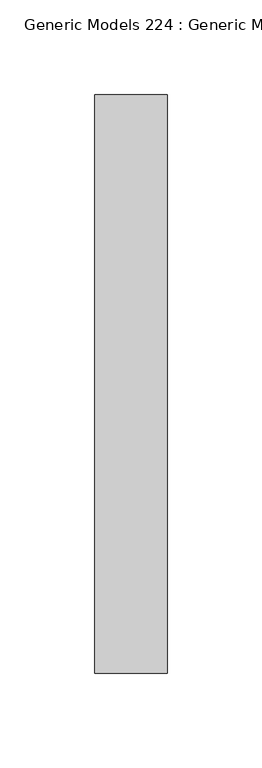
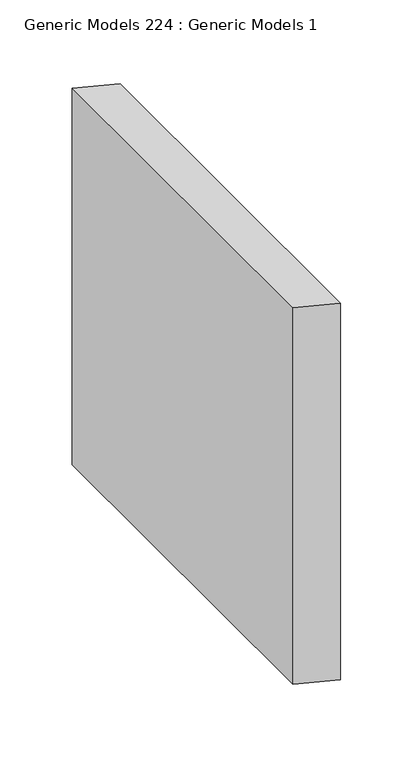
"""IFC4 building model written with IfcOpenShell, lengths in millimetres: proxy geometry, Generic Models 224 : Generic Models 1."""

from ifc_helpers import new_model, si_unit, frame, origin, place, context, project, spatial, polyline, outline, extrude, source, transform, mapped, element, save


def generic_models_224_generic_models_1_b6cca37e(model_context):
    return source(origin(), model_context, "Body", "SweptSolid", [
        extrude(outline(polyline([(126823.3589392, -31196.2089809), (126813.831285, -31158.1089809), (127131.3569728, -31158.1089809), (127140.8819728, -31196.2089809), (126823.3589392, -31196.2089809)])), frame((0.0, 21665.9639348, 0.0), z_axis=(0.0, 1.0, 0.0), x_axis=(0.0, 0.0, 1.0)), (0.0, 0.0, 1.0), 304.8),
    ])


if __name__ == "__main__":
    model = new_model("IFC4")
    model_context = context("Model", 3, world=origin())
    ifc_project = project(units=[si_unit("LENGTHUNIT", "METRE", prefix="MILLI")], contexts=[model_context])
    site = spatial("IfcSite", under=ifc_project)
    building = spatial("IfcBuilding", under=site)
    placement = place(None, origin())
    generic_models_224_generic_models_1_shape = generic_models_224_generic_models_1_b6cca37e(model_context)
    element("IfcBuildingElementProxy", 1, Name="Generic Models 224 : Generic Models 1", ObjectType="Generic Models 224 : Generic Models 1", at=placement, inside=building, context=model_context, shape_type="MappedRepresentation", body=[
        mapped(generic_models_224_generic_models_1_shape, transform((0.0, 0.0, 0.0), x_axis=(1.0, 0.0, 0.0), y_axis=(0.0, 1.0, 0.0), z_axis=(0.0, 0.0, 1.0))),
    ])
    save(model, "model.ifc")

# Revit data of these elements
# Element 1 (IfcBuildingElementProxy, "Generic Models 224 : Generic Models 1")
#   Materials on its faces: "_2X BLOCKING AS REQUIRED"
# Materials
#   "_2X BLOCKING AS REQUIRED": class "Generic", colour RGB 177 130 114, transparency 0, Cost = 0
